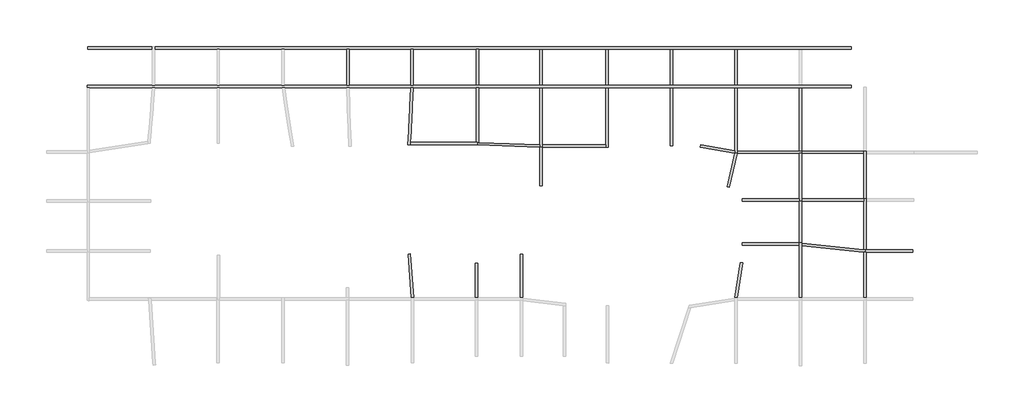
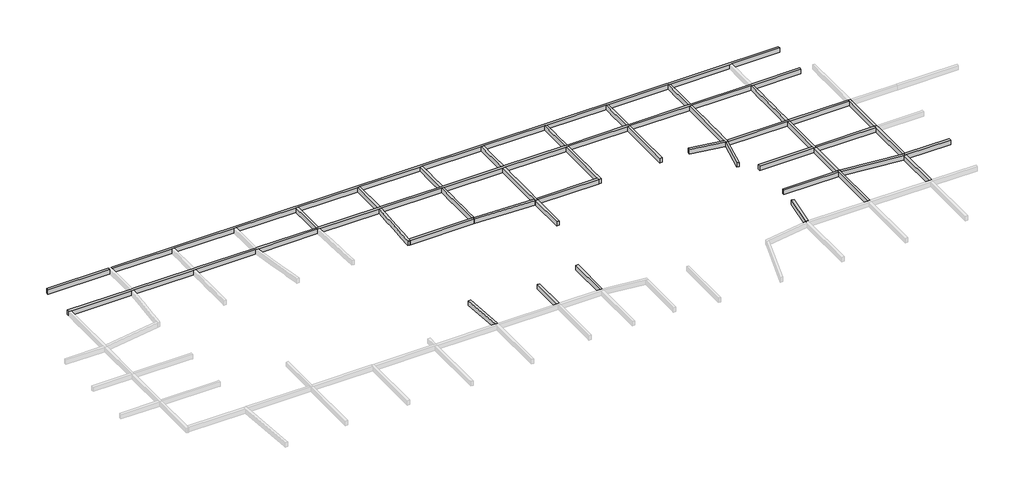
# One storey, part 7 of 8: 39 beams.
"""IFC4 building model written with IfcOpenShell, lengths in millimetres."""

from ifc_helpers import new_model, si_unit, frame, origin, place, context, project, spatial, polyline, outline, extrude, faceted_brep, element, save

model = new_model("IFC4")

# Units and contexts
model_context = context("Model", 3, world=origin())
ifc_project = project(units=[si_unit("LENGTHUNIT", "METRE", prefix="MILLI")], contexts=[model_context])

# Site, building, storey
site = spatial("IfcSite", under=ifc_project)
building = spatial("IfcBuilding", under=site)
storey = spatial("IfcBuildingStorey", under=building, Name="层高", Elevation=3300.0)

# Beams
placement = place(None, origin())
element("IfcBeam", 1, ObjectType="混凝土 - 矩形梁 : KL_beam", at=placement, inside=storey, context=model_context, shape_type="Brep", body=[
    faceted_brep([(155358.8476291, 153267.0451916, 3300.0), (155358.8476291, 152967.0451916, 3300.0), (155358.8476291, 152967.0451916, 2700.0), (155358.8476291, 153267.0451916, 2700.0), (149303.4366403, 153267.0451916, 3300.0), (149003.4366403, 153267.0451916, 3300.0), (141483.4366403, 153267.0451916, 3300.0), (141183.4366403, 153267.0451916, 3300.0), (133582.6046447, 153267.0451916, 3300.0), (133282.6046447, 153267.0451916, 3300.0), (125742.6046447, 153267.0451916, 3300.0), (125442.6046447, 153267.0451916, 3300.0), (117673.8474258, 153267.0451916, 3300.0), (117373.8474258, 153267.0451916, 3300.0), (109888.82396, 153267.0451916, 3300.0), (109588.82396, 153267.0451916, 3300.0), (101942.8755148, 153267.0451916, 3300.0), (101642.8755148, 153267.0451916, 3300.0), (94082.8755148, 153267.0451916, 3300.0), (93782.8755148, 153267.0451916, 3300.0), (86192.7452463, 153267.0451916, 3300.0), (85892.7452463, 153267.0451916, 3300.0), (78272.7452463, 153267.0451916, 3300.0), (77972.7452463, 153267.0451916, 3300.0), (70393.6976621, 153267.0451916, 3300.0), (70093.6976621, 153267.0451916, 3300.0), (62108.8476291, 153267.0451916, 3300.0), (62108.8476291, 152967.0451916, 3300.0), (62408.8476291, 152967.0451916, 3300.0), (70080.7837355, 152967.0451916, 3300.0), (70381.8074018, 152967.0451916, 3300.0), (77972.7452463, 152967.0451916, 3300.0), (78272.7452463, 152967.0451916, 3300.0), (85914.6331434, 152967.0451916, 3300.0), (86218.3726812, 152967.0451916, 3300.0), (93788.0221985, 152967.0451916, 3300.0), (94088.2050618, 152967.0451916, 3300.0), (101634.6906967, 152967.0451916, 3300.0), (101935.1141966, 152967.0451916, 3300.0), (109588.82396, 152967.0451916, 3300.0), (109888.82396, 152967.0451916, 3300.0), (117373.8474258, 152967.0451916, 3300.0), (117673.8474258, 152967.0451916, 3300.0), (125442.6046447, 152967.0451916, 3300.0), (125742.6046447, 152967.0451916, 3300.0), (133282.6046447, 152967.0451916, 3300.0), (133582.6046447, 152967.0451916, 3300.0), (141183.4366403, 152967.0451916, 3300.0), (141483.4366403, 152967.0451916, 3300.0), (149003.4366403, 152967.0451916, 3300.0), (149303.4366403, 152967.0451916, 3300.0), (62108.8476291, 152967.0451916, 2700.0), (62408.8476291, 152967.0451916, 2700.0), (70080.7837355, 152967.0451916, 2700.0), (70381.8074018, 152967.0451916, 2700.0), (77972.7452463, 152967.0451916, 2700.0), (78272.7452463, 152967.0451916, 2700.0), (85914.6331434, 152967.0451916, 2700.0), (86218.3726812, 152967.0451916, 2700.0), (93788.0221985, 152967.0451916, 2700.0), (94088.2050618, 152967.0451916, 2700.0), (101634.6906967, 152967.0451916, 2700.0), (101935.1141966, 152967.0451916, 2700.0), (109588.82396, 152967.0451916, 2700.0), (109888.82396, 152967.0451916, 2700.0), (117373.8474258, 152967.0451916, 2700.0), (117673.8474258, 152967.0451916, 2700.0), (125442.6046447, 152967.0451916, 2700.0), (125742.6046447, 152967.0451916, 2700.0), (133282.6046447, 152967.0451916, 2700.0), (133582.6046447, 152967.0451916, 2700.0), (141183.4366403, 152967.0451916, 2700.0), (141483.4366403, 152967.0451916, 2700.0), (149003.4366403, 152967.0451916, 2700.0), (149303.4366403, 152967.0451916, 2700.0), (62108.8476291, 153267.0451916, 2700.0), (70093.6976621, 153267.0451916, 2700.0), (70393.6976621, 153267.0451916, 2700.0), (77972.7452463, 153267.0451916, 2700.0), (78272.7452463, 153267.0451916, 2700.0), (85892.7452463, 153267.0451916, 2700.0), (86192.7452463, 153267.0451916, 2700.0), (93782.8755148, 153267.0451916, 2700.0), (94082.8755148, 153267.0451916, 2700.0), (101642.8755148, 153267.0451916, 2700.0), (101942.8755148, 153267.0451916, 2700.0), (109588.82396, 153267.0451916, 2700.0), (109888.82396, 153267.0451916, 2700.0), (117373.8474258, 153267.0451916, 2700.0), (117673.8474258, 153267.0451916, 2700.0), (125442.6046447, 153267.0451916, 2700.0), (125742.6046447, 153267.0451916, 2700.0), (133282.6046447, 153267.0451916, 2700.0), (133582.6046447, 153267.0451916, 2700.0), (141183.4366403, 153267.0451916, 2700.0), (141483.4366403, 153267.0451916, 2700.0), (149003.4366403, 153267.0451916, 2700.0), (149303.4366403, 153267.0451916, 2700.0)], [[[0, 1, 2, 3]], [[1, 0, 4, 5, 6, 7, 8, 9, 10, 11, 12, 13, 14, 15, 16, 17, 18, 19, 20, 21, 22, 23, 24, 25, 26, 27, 28, 29, 30, 31, 32, 33, 34, 35, 36, 37, 38, 39, 40, 41, 42, 43, 44, 45, 46, 47, 48, 49, 50]], [[2, 1, 50, 49, 48, 47, 46, 45, 44, 43, 42, 41, 40, 39, 38, 37, 36, 35, 34, 33, 32, 31, 30, 29, 28, 27, 51, 52, 53, 54, 55, 56, 57, 58, 59, 60, 61, 62, 63, 64, 65, 66, 67, 68, 69, 70, 71, 72, 73, 74]], [[3, 2, 74, 73, 72, 71, 70, 69, 68, 67, 66, 65, 64, 63, 62, 61, 60, 59, 58, 57, 56, 55, 54, 53, 52, 51, 75, 76, 77, 78, 79, 80, 81, 82, 83, 84, 85, 86, 87, 88, 89, 90, 91, 92, 93, 94, 95, 96, 97]], [[0, 3, 97, 96, 95, 94, 93, 92, 91, 90, 89, 88, 87, 86, 85, 84, 83, 82, 81, 80, 79, 78, 77, 76, 75, 26, 25, 24, 23, 22, 21, 20, 19, 18, 17, 16, 15, 14, 13, 12, 11, 10, 9, 8, 7, 6, 5, 4]], [[27, 26, 75, 51]]]),
])
element("IfcBeam", 2, ObjectType="混凝土 - 矩形梁 : KL_beam", at=placement, inside=storey, context=model_context, shape_type="Brep", body=[
    faceted_brep([(155398.8476291, 158006.8472847, 3300.0), (155398.8476291, 157706.8472847, 3300.0), (155398.8476291, 157706.8472847, 2700.0), (155398.8476291, 158006.8472847, 2700.0), (70393.6976621, 158006.8472847, 3300.0), (70393.6976621, 157706.8472847, 3300.0), (77972.7452463, 157706.8472847, 3300.0), (78272.7452463, 157706.8472847, 3300.0), (85892.7452463, 157706.8472847, 3300.0), (86192.7452463, 157706.8472847, 3300.0), (93782.8755148, 157706.8472847, 3300.0), (94082.8755148, 157706.8472847, 3300.0), (101642.8755148, 157706.8472847, 3300.0), (101942.8755148, 157706.8472847, 3300.0), (109588.82396, 157706.8472847, 3300.0), (109888.82396, 157706.8472847, 3300.0), (117373.8474258, 157706.8472847, 3300.0), (117673.8474258, 157706.8472847, 3300.0), (125442.6046447, 157706.8472847, 3300.0), (125742.6046447, 157706.8472847, 3300.0), (133282.6046447, 157706.8472847, 3300.0), (133582.6046447, 157706.8472847, 3300.0), (141183.4366403, 157706.8472847, 3300.0), (141483.4366403, 157706.8472847, 3300.0), (149003.4366403, 157706.8472847, 3300.0), (149303.4366403, 157706.8472847, 3300.0), (70393.6976621, 157706.8472847, 2700.0), (77972.7452463, 157706.8472847, 2700.0), (78272.7452463, 157706.8472847, 2700.0), (85892.7452463, 157706.8472847, 2700.0), (86192.7452463, 157706.8472847, 2700.0), (93782.8755148, 157706.8472847, 2700.0), (94082.8755148, 157706.8472847, 2700.0), (101642.8755148, 157706.8472847, 2700.0), (101942.8755148, 157706.8472847, 2700.0), (109588.82396, 157706.8472847, 2700.0), (109888.82396, 157706.8472847, 2700.0), (117373.8474258, 157706.8472847, 2700.0), (117673.8474258, 157706.8472847, 2700.0), (125442.6046447, 157706.8472847, 2700.0), (125742.6046447, 157706.8472847, 2700.0), (133282.6046447, 157706.8472847, 2700.0), (133582.6046447, 157706.8472847, 2700.0), (141183.4366403, 157706.8472847, 2700.0), (141483.4366403, 157706.8472847, 2700.0), (149003.4366403, 157706.8472847, 2700.0), (149303.4366403, 157706.8472847, 2700.0), (70393.6976621, 158006.8472847, 2700.0)], [[[0, 1, 2, 3]], [[1, 0, 4, 5, 6, 7, 8, 9, 10, 11, 12, 13, 14, 15, 16, 17, 18, 19, 20, 21, 22, 23, 24, 25]], [[2, 1, 25, 24, 23, 22, 21, 20, 19, 18, 17, 16, 15, 14, 13, 12, 11, 10, 9, 8, 7, 6, 5, 26, 27, 28, 29, 30, 31, 32, 33, 34, 35, 36, 37, 38, 39, 40, 41, 42, 43, 44, 45, 46]], [[3, 2, 46, 45, 44, 43, 42, 41, 40, 39, 38, 37, 36, 35, 34, 33, 32, 31, 30, 29, 28, 27, 26, 47]], [[0, 3, 47, 4]], [[5, 4, 47, 26]]]),
    faceted_brep([(62198.8476291, 158006.8472847, 3300.0), (62198.8476291, 158006.8472847, 2700.0), (62198.8476291, 157706.8472847, 2700.0), (62198.8476291, 157706.8472847, 3300.0), (70093.6976621, 158006.8472847, 3300.0), (70093.6976621, 157706.8472847, 3300.0), (70093.6976621, 157706.8472847, 2700.0), (70093.6976621, 158006.8472847, 2700.0)], [[[0, 1, 2, 3]], [[4, 5, 6, 7]], [[0, 3, 5, 4]], [[3, 2, 6, 5]], [[2, 1, 7, 6]], [[1, 0, 4, 7]]]),
])
element("IfcBeam", 3, ObjectType="混凝土 - 矩形梁 : KL_beam", at=placement, inside=storey, context=model_context, shape_type="Brep", body=[
    faceted_brep([(93782.8755148, 153267.0451916, 3300.0), (94082.8755148, 153267.0451916, 3300.0), (94082.8755148, 155366.9462381, 3300.0), (94082.8755148, 155766.9462381, 3300.0), (94082.8755148, 157706.8472847, 3300.0), (93782.8755148, 157706.8472847, 3300.0), (93782.8755148, 155766.9462381, 3300.0), (93782.8755148, 155366.9462381, 3300.0), (93782.8755148, 153267.0451916, 2700.0), (93782.8755148, 157706.8472847, 2700.0), (93782.8755148, 155766.9462381, 2700.0), (93782.8755148, 155366.9462381, 2700.0), (94082.8755148, 153267.0451916, 2700.0), (94082.8755148, 157706.8472847, 2700.0), (94082.8755148, 155766.9462381, 2700.0), (94082.8755148, 155366.9462381, 2700.0)], [[[0, 1, 2, 3, 4, 5, 6, 7]], [[8, 0, 7, 6, 5, 9, 10, 11]], [[12, 8, 11, 10, 9, 13, 14, 15]], [[1, 12, 15, 14, 13, 4, 3, 2]], [[1, 0, 8, 12]], [[5, 4, 13, 9]]]),
])
element("IfcBeam", 4, ObjectType="混凝土 - 矩形梁 : KL_beam", at=placement, inside=storey, context=model_context, shape_type="Brep", body=[
    faceted_brep([(101642.8755148, 153267.0451916, 3300.0), (101942.8755148, 153267.0451916, 3300.0), (101942.8755148, 155366.9462381, 3300.0), (101942.8755148, 155766.9462381, 3300.0), (101942.8755148, 157706.8472847, 3300.0), (101642.8755148, 157706.8472847, 3300.0), (101642.8755148, 155766.9462381, 3300.0), (101642.8755148, 155366.9462381, 3300.0), (101642.8755148, 153267.0451916, 2700.0), (101642.8755148, 157706.8472847, 2700.0), (101642.8755148, 155766.9462381, 2700.0), (101642.8755148, 155366.9462381, 2700.0), (101942.8755148, 153267.0451916, 2700.0), (101942.8755148, 157706.8472847, 2700.0), (101942.8755148, 155766.9462381, 2700.0), (101942.8755148, 155366.9462381, 2700.0)], [[[0, 1, 2, 3, 4, 5, 6, 7]], [[8, 0, 7, 6, 5, 9, 10, 11]], [[12, 8, 11, 10, 9, 13, 14, 15]], [[1, 12, 15, 14, 13, 4, 3, 2]], [[1, 0, 8, 12]], [[5, 4, 13, 9]]]),
])
element("IfcBeam", 5, ObjectType="混凝土 - 矩形梁 : KL_beam", at=placement, inside=storey, context=model_context, shape_type="Brep", body=[
    faceted_brep([(109588.82396, 153267.0451916, 3300.0), (109888.82396, 153267.0451916, 3300.0), (109888.82396, 155366.9462381, 3300.0), (109888.82396, 155766.9462381, 3300.0), (109888.82396, 157706.8472847, 3300.0), (109588.82396, 157706.8472847, 3300.0), (109588.82396, 155766.9462381, 3300.0), (109588.82396, 155366.9462381, 3300.0), (109588.82396, 153267.0451916, 2700.0), (109588.82396, 157706.8472847, 2700.0), (109588.82396, 155766.9462381, 2700.0), (109588.82396, 155366.9462381, 2700.0), (109888.82396, 153267.0451916, 2700.0), (109888.82396, 157706.8472847, 2700.0), (109888.82396, 155766.9462381, 2700.0), (109888.82396, 155366.9462381, 2700.0)], [[[0, 1, 2, 3, 4, 5, 6, 7]], [[8, 0, 7, 6, 5, 9, 10, 11]], [[12, 8, 11, 10, 9, 13, 14, 15]], [[1, 12, 15, 14, 13, 4, 3, 2]], [[1, 0, 8, 12]], [[5, 4, 13, 9]]]),
])
element("IfcBeam", 6, ObjectType="混凝土 - 矩形梁 : KL_beam", at=placement, inside=storey, context=model_context, shape_type="Brep", body=[
    faceted_brep([(117373.8474258, 153267.0451916, 3300.0), (117673.8474258, 153267.0451916, 3300.0), (117673.8474258, 155366.9462381, 3300.0), (117673.8474258, 155766.9462381, 3300.0), (117673.8474258, 157706.8472847, 3300.0), (117373.8474258, 157706.8472847, 3300.0), (117373.8474258, 155766.9462381, 3300.0), (117373.8474258, 155366.9462381, 3300.0), (117373.8474258, 153267.0451916, 2700.0), (117373.8474258, 157706.8472847, 2700.0), (117373.8474258, 155766.9462381, 2700.0), (117373.8474258, 155366.9462381, 2700.0), (117673.8474258, 153267.0451916, 2700.0), (117673.8474258, 157706.8472847, 2700.0), (117673.8474258, 155766.9462381, 2700.0), (117673.8474258, 155366.9462381, 2700.0)], [[[0, 1, 2, 3, 4, 5, 6, 7]], [[8, 0, 7, 6, 5, 9, 10, 11]], [[12, 8, 11, 10, 9, 13, 14, 15]], [[1, 12, 15, 14, 13, 4, 3, 2]], [[1, 0, 8, 12]], [[5, 4, 13, 9]]]),
])
element("IfcBeam", 7, ObjectType="混凝土 - 矩形梁 : KL_beam", at=placement, inside=storey, context=model_context, shape_type="Brep", body=[
    faceted_brep([(125442.6046447, 153267.0451916, 3300.0), (125742.6046447, 153267.0451916, 3300.0), (125742.6046447, 155366.9462381, 3300.0), (125742.6046447, 155766.9462381, 3300.0), (125742.6046447, 157706.8472847, 3300.0), (125442.6046447, 157706.8472847, 3300.0), (125442.6046447, 155766.9462381, 3300.0), (125442.6046447, 155366.9462381, 3300.0), (125442.6046447, 153267.0451916, 2700.0), (125442.6046447, 157706.8472847, 2700.0), (125442.6046447, 155766.9462381, 2700.0), (125442.6046447, 155366.9462381, 2700.0), (125742.6046447, 153267.0451916, 2700.0), (125742.6046447, 157706.8472847, 2700.0), (125742.6046447, 155766.9462381, 2700.0), (125742.6046447, 155366.9462381, 2700.0)], [[[0, 1, 2, 3, 4, 5, 6, 7]], [[8, 0, 7, 6, 5, 9, 10, 11]], [[12, 8, 11, 10, 9, 13, 14, 15]], [[1, 12, 15, 14, 13, 4, 3, 2]], [[1, 0, 8, 12]], [[5, 4, 13, 9]]]),
])
element("IfcBeam", 8, ObjectType="混凝土 - 矩形梁 : KL_beam", at=placement, inside=storey, context=model_context, shape_type="Brep", body=[
    faceted_brep([(133282.6046447, 153267.0451916, 3300.0), (133582.6046447, 153267.0451916, 3300.0), (133582.6046447, 155366.9462381, 3300.0), (133582.6046447, 155766.9462381, 3300.0), (133582.6046447, 157706.8472847, 3300.0), (133282.6046447, 157706.8472847, 3300.0), (133282.6046447, 155766.9462381, 3300.0), (133282.6046447, 155366.9462381, 3300.0), (133282.6046447, 153267.0451916, 2700.0), (133282.6046447, 157706.8472847, 2700.0), (133282.6046447, 155766.9462381, 2700.0), (133282.6046447, 155366.9462381, 2700.0), (133582.6046447, 153267.0451916, 2700.0), (133582.6046447, 157706.8472847, 2700.0), (133582.6046447, 155766.9462381, 2700.0), (133582.6046447, 155366.9462381, 2700.0)], [[[0, 1, 2, 3, 4, 5, 6, 7]], [[8, 0, 7, 6, 5, 9, 10, 11]], [[12, 8, 11, 10, 9, 13, 14, 15]], [[1, 12, 15, 14, 13, 4, 3, 2]], [[1, 0, 8, 12]], [[5, 4, 13, 9]]]),
])
element("IfcBeam", 9, ObjectType="混凝土 - 矩形梁 : KL_beam", at=placement, inside=storey, context=model_context, shape_type="Brep", body=[
    faceted_brep([(141183.4366403, 153267.0451916, 3300.0), (141483.4366403, 153267.0451916, 3300.0), (141483.4366403, 155366.9462381, 3300.0), (141483.4366403, 155766.9462381, 3300.0), (141483.4366403, 157706.8472847, 3300.0), (141183.4366403, 157706.8472847, 3300.0), (141183.4366403, 155766.9462381, 3300.0), (141183.4366403, 155366.9462381, 3300.0), (141183.4366403, 153267.0451916, 2700.0), (141183.4366403, 157706.8472847, 2700.0), (141183.4366403, 155766.9462381, 2700.0), (141183.4366403, 155366.9462381, 2700.0), (141483.4366403, 153267.0451916, 2700.0), (141483.4366403, 157706.8472847, 2700.0), (141483.4366403, 155766.9462381, 2700.0), (141483.4366403, 155366.9462381, 2700.0)], [[[0, 1, 2, 3, 4, 5, 6, 7]], [[8, 0, 7, 6, 5, 9, 10, 11]], [[12, 8, 11, 10, 9, 13, 14, 15]], [[1, 12, 15, 14, 13, 4, 3, 2]], [[1, 0, 8, 12]], [[5, 4, 13, 9]]]),
])
element("IfcBeam", 10, ObjectType="混凝土 - 矩形梁 : KL_beam", at=placement, inside=storey, context=model_context, shape_type="Brep", body=[
    faceted_brep([(101286.0486898, 132683.0858933, 3300.0), (101585.3179049, 132704.0128354, 3300.0), (101585.3179049, 132704.0128354, 2700.0), (101286.0486898, 132683.0858933, 2700.0), (101659.9672049, 127335.802002, 3300.0), (101670.8225114, 127335.802002, 3300.0), (101960.6997743, 127335.802002, 3300.0), (101960.6997743, 127335.802002, 2700.0), (101670.8225114, 127335.802002, 2700.0), (101659.9672049, 127335.802002, 2700.0)], [[[0, 1, 2, 3]], [[1, 0, 4, 5, 6]], [[2, 1, 6, 7]], [[3, 2, 7, 8, 9]], [[0, 3, 9, 4]], [[4, 9, 8, 7, 6, 5]]]),
    faceted_brep([(101981.6778179, 127035.802002, 2700.0), (101981.6778179, 127035.802002, 3300.0), (101970.8225114, 127035.802002, 3300.0), (101970.8225114, 127035.802002, 2700.0), (101970.8225114, 127191.0401174, 3300.0), (101970.8225114, 127191.0401174, 2700.0)], [[[0, 1, 2, 3]], [[2, 4, 5, 3]], [[1, 4, 2]], [[1, 0, 5, 4]], [[5, 0, 3]]]),
])
element("IfcBeam", 11, ObjectType="混凝土 - 矩形梁 : KL_beam", at=placement, inside=storey, context=model_context, shape_type="SweptSolid", body=[
    extrude(outline(polyline([(109470.8225114, 131593.2738066), (109770.8225114, 131593.2738066), (109770.8225114, 127335.802002), (109470.8225114, 127335.802002), (109470.8225114, 131593.2738066)])), frame((0.0, 0.0, 2700.0), z_axis=(0.0, 0.0, 1.0), x_axis=(1.0, 0.0, 0.0)), (0.0, 0.0, 1.0), 600.0),
])
element("IfcBeam", 12, ObjectType="混凝土 - 矩形梁 : KL_beam", at=placement, inside=storey, context=model_context, shape_type="SweptSolid", body=[
    extrude(outline(polyline([(114973.8238915, 132693.2738046), (115273.8238915, 132693.2738046), (115273.8238915, 127335.802002), (114973.8238915, 127335.802002), (114973.8238915, 132693.2738046)])), frame((0.0, 0.0, 2700.0), z_axis=(0.0, 0.0, 1.0), x_axis=(1.0, 0.0, 0.0)), (0.0, 0.0, 1.0), 600.0),
])
element("IfcBeam", 13, ObjectType="混凝土 - 矩形梁 : KL_beam", at=placement, inside=storey, context=model_context, shape_type="Brep", body=[
    faceted_brep([(149348.8238805, 134044.1147453, 3300.0), (149303.4366403, 134044.1147453, 3300.0), (149206.6850474, 134044.1147453, 3300.0), (149048.8238805, 134044.1147453, 3300.0), (149048.8238805, 133744.1147453, 3300.0), (149048.8238805, 127344.1147453, 3300.0), (149348.8238805, 127344.1147453, 3300.0), (149348.8238805, 133727.5228681, 3300.0), (149348.8238805, 134029.175352, 3300.0), (149348.8238805, 134044.1147453, 2700.0), (149348.8238805, 127344.1147453, 2700.0), (149348.8238805, 133727.5228681, 2700.0), (149348.8238805, 134029.175352, 2700.0), (149048.8238805, 134044.1147453, 2700.0), (149206.6850474, 134044.1147453, 2700.0), (149303.4366403, 134044.1147453, 2700.0), (149048.8238805, 127344.1147453, 2700.0), (149048.8238805, 133744.1147453, 2700.0)], [[[0, 1, 2, 3, 4, 5, 6, 7, 8]], [[9, 0, 8, 7, 6, 10, 11, 12]], [[13, 14, 15, 9, 12, 11, 10, 16, 17]], [[3, 13, 17, 16, 5, 4]], [[6, 5, 16, 10]], [[3, 2, 1, 0, 9, 15, 14, 13]]]),
])
element("IfcBeam", 14, ObjectType="混凝土 - 矩形梁 : KL_beam", at=placement, inside=storey, context=model_context, shape_type="Brep", body=[
    faceted_brep([(141854.6257221, 131662.1774478, 3300.0), (142150.9322243, 131615.2471082, 3300.0), (142150.9322243, 131615.2471082, 2700.0), (141854.6257221, 131662.1774478, 2700.0), (141170.7117777, 127344.1147453, 3300.0), (141448.8238805, 127344.1147453, 3300.0), (141474.4513154, 127344.1147453, 3300.0), (141474.4513154, 127344.1147453, 2700.0), (141448.8238805, 127344.1147453, 2700.0), (141170.7117777, 127344.1147453, 2700.0)], [[[0, 1, 2, 3]], [[1, 0, 4, 5, 6]], [[2, 1, 6, 7]], [[3, 2, 7, 8, 9]], [[0, 3, 9, 4]], [[4, 9, 8, 7, 6, 5]]]),
    faceted_brep([(141118.3137403, 127013.2865575, 3300.0), (141118.3137403, 127013.2865575, 2700.0), (141148.8238805, 127018.1739614, 2700.0), (141148.8238805, 127018.1739614, 3300.0), (141148.8238805, 127205.9200013, 2700.0), (141148.8238805, 127205.9200013, 3300.0), (141148.8238805, 127044.1147453, 3300.0), (141148.8238805, 127044.1147453, 2700.0)], [[[0, 1, 2, 3]], [[4, 5, 6, 3, 2, 7]], [[5, 0, 3, 6]], [[1, 4, 7, 2]], [[1, 0, 5, 4]]]),
])
element("IfcBeam", 15, ObjectType="混凝土 - 矩形梁 : KL_beam", at=placement, inside=storey, context=model_context, shape_type="Brep", body=[
    faceted_brep([(142092.714265, 133744.1147453, 3300.0), (142092.714265, 134044.1147453, 3300.0), (142092.714265, 134044.1147453, 2700.0), (142092.714265, 133744.1147453, 2700.0), (149048.8238805, 133744.1147453, 3300.0), (149048.8238805, 134044.1147453, 3300.0), (149044.6739148, 134044.1147453, 3300.0), (149003.4366403, 134044.1147453, 3300.0), (149048.8238805, 134044.1147453, 2700.0), (149044.6739148, 134044.1147453, 2700.0), (149003.4366403, 134044.1147453, 2700.0), (149048.8238805, 133744.1147453, 2700.0)], [[[0, 1, 2, 3]], [[1, 0, 4, 5, 6, 7]], [[2, 1, 7, 6, 5, 8, 9, 10]], [[3, 2, 10, 9, 8, 11]], [[0, 3, 11, 4]], [[5, 4, 11, 8]]]),
])
element("IfcBeam", 16, ObjectType="混凝土 - 矩形梁 : KL_beam", at=placement, inside=storey, context=model_context, shape_type="Brep", body=[
    faceted_brep([(149348.8238805, 133727.5228681, 3300.0), (156905.5468539, 132933.2792789, 3300.0), (157047.685687, 132918.3398855, 3300.0), (157063.4080208, 133218.3398855, 3300.0), (156905.5468539, 133234.9317627, 3300.0), (149348.8238805, 134029.175352, 3300.0), (149348.8238805, 133744.1147453, 3300.0), (149348.8238805, 133727.5228681, 2700.0), (156905.5468539, 132933.2792789, 2700.0), (157047.685687, 132918.3398855, 2700.0), (149348.8238805, 133744.1147453, 2700.0), (149348.8238805, 134029.175352, 2700.0), (156905.5468539, 133234.9317627, 2700.0), (157063.4080208, 133218.3398855, 2700.0)], [[[0, 1, 2, 3, 4, 5, 6]], [[2, 1, 0, 7, 8, 9]], [[9, 8, 7, 10, 11, 12, 13]], [[11, 5, 4, 3, 13, 12]], [[7, 0, 6, 5, 11, 10]], [[3, 2, 9, 13]]]),
    faceted_brep([(149046.4440807, 134060.9567496, 3300.0), (149046.4440807, 134060.9567496, 2700.0), (149044.6739148, 134044.1147453, 2700.0), (149044.6739148, 134044.1147453, 3300.0), (149048.8238805, 134044.1147453, 2700.0), (149206.6850474, 134044.1147453, 2700.0), (149206.6850474, 134044.1147453, 3300.0), (149048.8238805, 134044.1147453, 3300.0)], [[[0, 1, 2, 3]], [[3, 2, 4, 5, 6, 7]], [[3, 7, 6, 0]], [[5, 4, 2, 1]], [[1, 0, 6, 5]]]),
])
element("IfcBeam", 17, ObjectType="混凝土 - 矩形梁 : KL_beam", at=placement, inside=storey, context=model_context, shape_type="Brep", body=[
    faceted_brep([(162873.6972933, 133218.3398855, 3300.0), (162873.6972933, 132918.3398855, 3300.0), (162873.6972933, 132918.3398855, 2700.0), (162873.6972933, 133218.3398855, 2700.0), (157205.5468539, 133218.3398855, 3300.0), (157063.4080208, 133218.3398855, 3300.0), (157047.685687, 132918.3398855, 3300.0), (157205.5468539, 132918.3398855, 3300.0), (157047.685687, 132918.3398855, 2700.0), (157205.5468539, 132918.3398855, 2700.0), (157063.4080208, 133218.3398855, 2700.0), (157205.5468539, 133218.3398855, 2700.0)], [[[0, 1, 2, 3]], [[1, 0, 4, 5, 6, 7]], [[2, 1, 7, 6, 8, 9]], [[3, 2, 9, 8, 10, 11]], [[0, 3, 11, 10, 5, 4]], [[5, 10, 8, 6]]]),
])
element("IfcBeam", 18, ObjectType="混凝土 - 矩形梁 : KL_beam", at=placement, inside=storey, context=model_context, shape_type="SweptSolid", body=[
    extrude(outline(polyline([(157205.5468539, 127344.1147453), (156905.5468539, 127344.1147453), (156905.5468539, 132933.2792789), (157047.685687, 132918.3398855), (157205.5468539, 132918.3398855), (157205.5468539, 127344.1147453)])), frame((0.0, 0.0, 2700.0), z_axis=(0.0, 0.0, 1.0), x_axis=(1.0, 0.0, 0.0)), (0.0, 0.0, 1.0), 600.0),
])
element("IfcBeam", 19, ObjectType="混凝土 - 矩形梁 : KL_beam", at=placement, inside=storey, context=model_context, shape_type="Brep", body=[
    faceted_brep([(156905.5468539, 133234.9317627, 3300.0), (157063.4080208, 133218.3398855, 3300.0), (157205.5468539, 133218.3398855, 3300.0), (157205.5468539, 139118.3398855, 3300.0), (157205.5468539, 139418.3398855, 3300.0), (156905.5468539, 139418.3398855, 3300.0), (156905.5468539, 139118.3398855, 3300.0), (157205.5468539, 133218.3398855, 2700.0), (157205.5468539, 139118.3398855, 2700.0), (157205.5468539, 139418.3398855, 2700.0), (157063.4080208, 133218.3398855, 2700.0), (156905.5468539, 133234.9317627, 2700.0), (156905.5468539, 139118.3398855, 2700.0), (156905.5468539, 139418.3398855, 2700.0)], [[[0, 1, 2, 3, 4, 5, 6]], [[2, 7, 8, 9, 4, 3]], [[10, 11, 12, 13, 9, 8, 7]], [[11, 0, 6, 5, 13, 12]], [[1, 0, 11, 10]], [[2, 1, 10, 7]], [[5, 4, 9, 13]]]),
])
element("IfcBeam", 20, ObjectType="混凝土 - 矩形梁 : KL_beam", at=placement, inside=storey, context=model_context, shape_type="Brep", body=[
    faceted_brep([(157205.5468539, 145218.3398855, 3300.0), (156905.5468539, 145218.3398855, 3300.0), (156905.5468539, 144967.0451916, 3300.0), (156905.5468539, 139418.3398855, 3300.0), (157205.5468539, 139418.3398855, 3300.0), (157205.5468539, 144918.3398855, 3300.0), (157205.5468539, 145218.3398855, 2700.0), (157205.5468539, 139418.3398855, 2700.0), (157205.5468539, 144918.3398855, 2700.0), (156905.5468539, 145218.3398855, 2700.0), (156905.5468539, 139418.3398855, 2700.0), (156905.5468539, 144967.0451916, 2700.0)], [[[0, 1, 2, 3, 4, 5]], [[6, 0, 5, 4, 7, 8]], [[9, 6, 8, 7, 10, 11]], [[1, 9, 11, 10, 3, 2]], [[1, 0, 6, 9]], [[4, 3, 10, 7]]]),
])
element("IfcBeam", 21, ObjectType="混凝土 - 矩形梁 : KL_beam", at=placement, inside=storey, context=model_context, shape_type="Brep", body=[
    faceted_brep([(101265.6115787, 146023.4361595, 3300.0), (101565.1886759, 146007.5125022, 3300.0), (101581.1348121, 146307.5125022, 3300.0), (101652.7187262, 147654.2446479, 3300.0), (101673.9802411, 148054.2446479, 3300.0), (101799.0194755, 150406.6496336, 3300.0), (101820.2809905, 150806.6496336, 3300.0), (101935.1141966, 152967.0451916, 3300.0), (101634.6906967, 152967.0451916, 3300.0), (101519.8574906, 150806.6496336, 3300.0), (101498.5959757, 150406.6496336, 3300.0), (101373.5567413, 148054.2446479, 3300.0), (101352.2952263, 147654.2446479, 3300.0), (101265.6115787, 146023.4361595, 2700.0), (101634.6906967, 152967.0451916, 2700.0), (101519.8574906, 150806.6496336, 2700.0), (101498.5959757, 150406.6496336, 2700.0), (101373.5567413, 148054.2446479, 2700.0), (101352.2952263, 147654.2446479, 2700.0), (101565.1886759, 146007.5125022, 2700.0), (101935.1141966, 152967.0451916, 2700.0), (101820.2809905, 150806.6496336, 2700.0), (101799.0194755, 150406.6496336, 2700.0), (101673.9802411, 148054.2446479, 2700.0), (101652.7187262, 147654.2446479, 2700.0), (101581.1348121, 146307.5125022, 2700.0)], [[[0, 1, 2, 3, 4, 5, 6, 7, 8, 9, 10, 11, 12]], [[13, 0, 12, 11, 10, 9, 8, 14, 15, 16, 17, 18]], [[19, 13, 18, 17, 16, 15, 14, 20, 21, 22, 23, 24, 25]], [[1, 19, 25, 24, 23, 22, 21, 20, 7, 6, 5, 4, 3, 2]], [[8, 7, 20, 14]], [[1, 0, 13, 19]]]),
])
element("IfcBeam", 22, ObjectType="混凝土 - 矩形梁 : KL_beam", at=placement, inside=storey, context=model_context, shape_type="Brep", body=[
    faceted_brep([(109888.82396, 152967.0451916, 3300.0), (109588.82396, 152967.0451916, 3300.0), (109588.82396, 150806.6496336, 3300.0), (109588.82396, 150406.6496336, 3300.0), (109588.82396, 148054.2446479, 3300.0), (109588.82396, 147654.2446479, 3300.0), (109588.82396, 146307.5125022, 3300.0), (109731.2172347, 146307.5125022, 3300.0), (109888.82396, 146302.0087541, 3300.0), (109888.82396, 147654.2446479, 3300.0), (109888.82396, 148054.2446479, 3300.0), (109888.82396, 150406.6496336, 3300.0), (109888.82396, 150806.6496336, 3300.0), (109588.82396, 152967.0451916, 2700.0), (109588.82396, 150806.6496336, 2700.0), (109588.82396, 150406.6496336, 2700.0), (109588.82396, 148054.2446479, 2700.0), (109588.82396, 147654.2446479, 2700.0), (109588.82396, 146307.5125022, 2700.0), (109888.82396, 152967.0451916, 2700.0), (109888.82396, 150806.6496336, 2700.0), (109888.82396, 150406.6496336, 2700.0), (109888.82396, 148054.2446479, 2700.0), (109888.82396, 147654.2446479, 2700.0), (109888.82396, 146302.0087541, 2700.0), (109731.2172347, 146307.5125022, 2700.0)], [[[0, 1, 2, 3, 4, 5, 6, 7, 8, 9, 10, 11, 12]], [[1, 13, 14, 15, 16, 17, 18, 6, 5, 4, 3, 2]], [[13, 19, 20, 21, 22, 23, 24, 25, 18, 17, 16, 15, 14]], [[19, 0, 12, 11, 10, 9, 8, 24, 23, 22, 21, 20]], [[1, 0, 19, 13]], [[8, 7, 25, 24]], [[7, 6, 18, 25]]]),
])
element("IfcBeam", 23, ObjectType="混凝土 - 矩形梁 : KL_beam", at=placement, inside=storey, context=model_context, shape_type="Brep", body=[
    faceted_brep([(117373.8474258, 145735.2964279, 3300.0), (117673.8474258, 145735.2964279, 3300.0), (117673.8474258, 146035.2964279, 3300.0), (117673.8474258, 147654.2446479, 3300.0), (117673.8474258, 148054.2446479, 3300.0), (117673.8474258, 150406.6496336, 3300.0), (117673.8474258, 150806.6496336, 3300.0), (117673.8474258, 152967.0451916, 3300.0), (117373.8474258, 152967.0451916, 3300.0), (117373.8474258, 150806.6496336, 3300.0), (117373.8474258, 150406.6496336, 3300.0), (117373.8474258, 148054.2446479, 3300.0), (117373.8474258, 147654.2446479, 3300.0), (117373.8474258, 146040.625975, 3300.0), (117373.8474258, 145740.4431117, 3300.0), (117373.8474258, 145735.2964279, 2700.0), (117373.8474258, 152967.0451916, 2700.0), (117373.8474258, 150806.6496336, 2700.0), (117373.8474258, 150406.6496336, 2700.0), (117373.8474258, 148054.2446479, 2700.0), (117373.8474258, 147654.2446479, 2700.0), (117373.8474258, 146040.625975, 2700.0), (117373.8474258, 145740.4431117, 2700.0), (117673.8474258, 145735.2964279, 2700.0), (117673.8474258, 152967.0451916, 2700.0), (117673.8474258, 150806.6496336, 2700.0), (117673.8474258, 150406.6496336, 2700.0), (117673.8474258, 148054.2446479, 2700.0), (117673.8474258, 147654.2446479, 2700.0), (117673.8474258, 146035.2964279, 2700.0)], [[[0, 1, 2, 3, 4, 5, 6, 7, 8, 9, 10, 11, 12, 13, 14]], [[15, 0, 14, 13, 12, 11, 10, 9, 8, 16, 17, 18, 19, 20, 21, 22]], [[23, 15, 22, 21, 20, 19, 18, 17, 16, 24, 25, 26, 27, 28, 29]], [[1, 23, 29, 28, 27, 26, 25, 24, 7, 6, 5, 4, 3, 2]], [[8, 7, 24, 16]], [[1, 0, 15, 23]]]),
])
element("IfcBeam", 24, ObjectType="混凝土 - 矩形梁 : KL_beam", at=placement, inside=storey, context=model_context, shape_type="SweptSolid", body=[
    extrude(outline(polyline([(117673.8474258, 141044.2705383), (117373.8474258, 141044.2705383), (117373.8474258, 145735.2964279), (117673.8474258, 145735.2964279), (117673.8474258, 141044.2705383)])), frame((0.0, 0.0, 2700.0), z_axis=(0.0, 0.0, 1.0), x_axis=(1.0, 0.0, 0.0)), (0.0, 0.0, 1.0), 600.0),
])
element("IfcBeam", 25, ObjectType="混凝土 - 矩形梁 : KL_beam", at=placement, inside=storey, context=model_context, shape_type="Brep", body=[
    faceted_brep([(125442.6046447, 145735.2964279, 3300.0), (125742.6046447, 145735.2964279, 3300.0), (125742.6046447, 147654.2446479, 3300.0), (125742.6046447, 148054.2446479, 3300.0), (125742.6046447, 150406.6496336, 3300.0), (125742.6046447, 150806.6496336, 3300.0), (125742.6046447, 152967.0451916, 3300.0), (125442.6046447, 152967.0451916, 3300.0), (125442.6046447, 150806.6496336, 3300.0), (125442.6046447, 150406.6496336, 3300.0), (125442.6046447, 148054.2446479, 3300.0), (125442.6046447, 147654.2446479, 3300.0), (125442.6046447, 146035.2964279, 3300.0), (125442.6046447, 145735.2964279, 2700.0), (125442.6046447, 152967.0451916, 2700.0), (125442.6046447, 150806.6496336, 2700.0), (125442.6046447, 150406.6496336, 2700.0), (125442.6046447, 148054.2446479, 2700.0), (125442.6046447, 147654.2446479, 2700.0), (125442.6046447, 146035.2964279, 2700.0), (125742.6046447, 145735.2964279, 2700.0), (125742.6046447, 152967.0451916, 2700.0), (125742.6046447, 150806.6496336, 2700.0), (125742.6046447, 150406.6496336, 2700.0), (125742.6046447, 148054.2446479, 2700.0), (125742.6046447, 147654.2446479, 2700.0)], [[[0, 1, 2, 3, 4, 5, 6, 7, 8, 9, 10, 11, 12]], [[13, 0, 12, 11, 10, 9, 8, 7, 14, 15, 16, 17, 18, 19]], [[20, 13, 19, 18, 17, 16, 15, 14, 21, 22, 23, 24, 25]], [[1, 20, 25, 24, 23, 22, 21, 6, 5, 4, 3, 2]], [[7, 6, 21, 14]], [[1, 0, 13, 20]]]),
])
element("IfcBeam", 26, ObjectType="混凝土 - 矩形梁 : KL_beam", at=placement, inside=storey, context=model_context, shape_type="Brep", body=[
    faceted_brep([(133582.6046447, 145885.6708097, 3300.0), (133282.6046447, 145885.6708097, 3300.0), (133282.6046447, 145885.6708097, 2700.0), (133582.6046447, 145885.6708097, 2700.0), (133582.6046447, 147654.2446479, 3300.0), (133582.6046447, 148054.2446479, 3300.0), (133582.6046447, 150406.6496336, 3300.0), (133582.6046447, 150806.6496336, 3300.0), (133582.6046447, 152967.0451916, 3300.0), (133282.6046447, 152967.0451916, 3300.0), (133282.6046447, 150806.6496336, 3300.0), (133282.6046447, 150406.6496336, 3300.0), (133282.6046447, 148054.2446479, 3300.0), (133282.6046447, 147654.2446479, 3300.0), (133282.6046447, 152967.0451916, 2700.0), (133282.6046447, 150806.6496336, 2700.0), (133282.6046447, 150406.6496336, 2700.0), (133282.6046447, 148054.2446479, 2700.0), (133282.6046447, 147654.2446479, 2700.0), (133582.6046447, 152967.0451916, 2700.0), (133582.6046447, 150806.6496336, 2700.0), (133582.6046447, 150406.6496336, 2700.0), (133582.6046447, 148054.2446479, 2700.0), (133582.6046447, 147654.2446479, 2700.0)], [[[0, 1, 2, 3]], [[1, 0, 4, 5, 6, 7, 8, 9, 10, 11, 12, 13]], [[2, 1, 13, 12, 11, 10, 9, 14, 15, 16, 17, 18]], [[3, 2, 18, 17, 16, 15, 14, 19, 20, 21, 22, 23]], [[0, 3, 23, 22, 21, 20, 19, 8, 7, 6, 5, 4]], [[9, 8, 19, 14]]]),
])
element("IfcBeam", 27, ObjectType="混凝土 - 矩形梁 : KL_beam", at=placement, inside=storey, context=model_context, shape_type="Brep", body=[
    faceted_brep([(141183.4366403, 144991.2614678, 3300.0), (141483.4366403, 144991.2614678, 3300.0), (141483.4366403, 145267.0451916, 3300.0), (141483.4366403, 147654.2446479, 3300.0), (141483.4366403, 148054.2446479, 3300.0), (141483.4366403, 150406.6496336, 3300.0), (141483.4366403, 150806.6496336, 3300.0), (141483.4366403, 152967.0451916, 3300.0), (141183.4366403, 152967.0451916, 3300.0), (141183.4366403, 150806.6496336, 3300.0), (141183.4366403, 150406.6496336, 3300.0), (141183.4366403, 148054.2446479, 3300.0), (141183.4366403, 147654.2446479, 3300.0), (141183.4366403, 145295.9236611, 3300.0), (141183.4366403, 144991.2614678, 2700.0), (141183.4366403, 152967.0451916, 2700.0), (141183.4366403, 150806.6496336, 2700.0), (141183.4366403, 150406.6496336, 2700.0), (141183.4366403, 148054.2446479, 2700.0), (141183.4366403, 147654.2446479, 2700.0), (141183.4366403, 145295.9236611, 2700.0), (141483.4366403, 144991.2614678, 2700.0), (141483.4366403, 152967.0451916, 2700.0), (141483.4366403, 150806.6496336, 2700.0), (141483.4366403, 150406.6496336, 2700.0), (141483.4366403, 148054.2446479, 2700.0), (141483.4366403, 147654.2446479, 2700.0), (141483.4366403, 145267.0451916, 2700.0)], [[[0, 1, 2, 3, 4, 5, 6, 7, 8, 9, 10, 11, 12, 13]], [[14, 0, 13, 12, 11, 10, 9, 8, 15, 16, 17, 18, 19, 20]], [[21, 14, 20, 19, 18, 17, 16, 15, 22, 23, 24, 25, 26, 27]], [[1, 21, 27, 26, 25, 24, 23, 22, 7, 6, 5, 4, 3, 2]], [[8, 7, 22, 15]], [[1, 0, 14, 21]]]),
])
element("IfcBeam", 28, ObjectType="混凝土 - 矩形梁 : KL_beam", at=placement, inside=storey, context=model_context, shape_type="Brep", body=[
    faceted_brep([(137018.8891994, 146032.9756187, 3300.0), (137018.8891994, 146032.9756187, 2700.0), (136966.6069535, 145737.5664673, 2700.0), (136966.6069535, 145737.5664673, 3300.0), (141151.7464142, 144996.8700828, 3300.0), (141183.4366403, 144991.2614678, 3300.0), (141183.4366403, 145295.9236611, 3300.0), (141151.7464142, 144996.8700828, 2700.0), (141183.4366403, 144991.2614678, 2700.0), (141183.4366403, 145295.9236611, 2700.0)], [[[0, 1, 2, 3]], [[0, 3, 4, 5, 6]], [[3, 2, 7, 8, 5, 4]], [[2, 1, 9, 8, 7]], [[1, 0, 6, 9]], [[6, 5, 8, 9]]]),
])
element("IfcBeam", 29, ObjectType="混凝土 - 矩形梁 : KL_beam", at=placement, inside=storey, context=model_context, shape_type="Brep", body=[
    faceted_brep([(141483.4366403, 144991.2614678, 3300.0), (141183.4366403, 144991.2614678, 3300.0), (141151.7464142, 144996.8700828, 3300.0), (141144.8607955, 144967.0451916, 3300.0), (141452.7520278, 144967.0451916, 3300.0), (149003.4366403, 144967.0451916, 3300.0), (149303.4366403, 144967.0451916, 3300.0), (149303.4366403, 145267.0451916, 3300.0), (149003.4366403, 145267.0451916, 3300.0), (141483.4366403, 145267.0451916, 3300.0), (141483.4366403, 145242.8289154, 3300.0), (141144.8607955, 144967.0451916, 2700.0), (141452.7520278, 144967.0451916, 2700.0), (149003.4366403, 144967.0451916, 2700.0), (149303.4366403, 144967.0451916, 2700.0), (141183.4366403, 144991.2614678, 2700.0), (141483.4366403, 144991.2614678, 2700.0), (141483.4366403, 145242.8289154, 2700.0), (141483.4366403, 145267.0451916, 2700.0), (149003.4366403, 145267.0451916, 2700.0), (149303.4366403, 145267.0451916, 2700.0), (141151.7464142, 144996.8700828, 2700.0)], [[[0, 1, 2, 3, 4, 5, 6, 7, 8, 9, 10]], [[3, 11, 12, 13, 14, 6, 5, 4]], [[15, 16, 17, 18, 19, 20, 14, 13, 12, 11, 21]], [[18, 9, 8, 7, 20, 19]], [[11, 3, 2, 21]], [[16, 0, 10, 9, 18, 17]], [[0, 16, 15, 1]], [[2, 1, 15, 21]], [[7, 6, 14, 20]]]),
])
element("IfcBeam", 30, ObjectType="混凝土 - 矩形梁 : KL_beam", at=placement, inside=storey, context=model_context, shape_type="Brep", body=[
    faceted_brep([(156905.5468539, 144967.0451916, 3300.0), (156905.5468539, 145218.3398855, 3300.0), (156905.5468539, 145267.0451916, 3300.0), (149303.4366403, 145267.0451916, 3300.0), (149303.4366403, 144967.0451916, 3300.0), (156905.5468539, 144967.0451916, 2700.0), (149303.4366403, 144967.0451916, 2700.0), (156905.5468539, 145267.0451916, 2700.0), (156905.5468539, 145218.3398855, 2700.0), (149303.4366403, 145267.0451916, 2700.0)], [[[0, 1, 2, 3, 4]], [[5, 0, 4, 6]], [[7, 8, 5, 6, 9]], [[2, 7, 9, 3]], [[0, 5, 8, 7, 2, 1]], [[4, 3, 9, 6]]]),
])
element("IfcBeam", 31, ObjectType="混凝土 - 矩形梁 : KL_beam", at=placement, inside=storey, context=model_context, shape_type="Brep", body=[
    faceted_brep([(149003.4366403, 145267.0451916, 3300.0), (149303.4366403, 145267.0451916, 3300.0), (149303.4366403, 147654.2446479, 3300.0), (149303.4366403, 148054.2446479, 3300.0), (149303.4366403, 150406.6496336, 3300.0), (149303.4366403, 150806.6496336, 3300.0), (149303.4366403, 152967.0451916, 3300.0), (149003.4366403, 152967.0451916, 3300.0), (149003.4366403, 150806.6496336, 3300.0), (149003.4366403, 150406.6496336, 3300.0), (149003.4366403, 148054.2446479, 3300.0), (149003.4366403, 147654.2446479, 3300.0), (149003.4366403, 145267.0451916, 2700.0), (149003.4366403, 152967.0451916, 2700.0), (149003.4366403, 150806.6496336, 2700.0), (149003.4366403, 150406.6496336, 2700.0), (149003.4366403, 148054.2446479, 2700.0), (149003.4366403, 147654.2446479, 2700.0), (149303.4366403, 145267.0451916, 2700.0), (149303.4366403, 152967.0451916, 2700.0), (149303.4366403, 150806.6496336, 2700.0), (149303.4366403, 150406.6496336, 2700.0), (149303.4366403, 148054.2446479, 2700.0), (149303.4366403, 147654.2446479, 2700.0)], [[[0, 1, 2, 3, 4, 5, 6, 7, 8, 9, 10, 11]], [[12, 0, 11, 10, 9, 8, 7, 13, 14, 15, 16, 17]], [[18, 12, 17, 16, 15, 14, 13, 19, 20, 21, 22, 23]], [[1, 18, 23, 22, 21, 20, 19, 6, 5, 4, 3, 2]], [[1, 0, 12, 18]], [[7, 6, 19, 13]]]),
])
element("IfcBeam", 32, ObjectType="混凝土 - 矩形梁 : KL_beam", at=placement, inside=storey, context=model_context, shape_type="Brep", body=[
    faceted_brep([(149003.4366403, 139118.3398855, 3300.0), (149303.4366403, 139118.3398855, 3300.0), (149303.4366403, 139418.3398855, 3300.0), (149303.4366403, 144967.0451916, 3300.0), (149003.4366403, 144967.0451916, 3300.0), (149003.4366403, 139418.3398855, 3300.0), (149003.4366403, 139118.3398855, 2700.0), (149003.4366403, 144967.0451916, 2700.0), (149003.4366403, 139418.3398855, 2700.0), (149303.4366403, 139118.3398855, 2700.0), (149303.4366403, 144967.0451916, 2700.0), (149303.4366403, 139418.3398855, 2700.0)], [[[0, 1, 2, 3, 4, 5]], [[6, 0, 5, 4, 7, 8]], [[9, 6, 8, 7, 10, 11]], [[1, 9, 11, 10, 3, 2]], [[4, 3, 10, 7]], [[1, 0, 6, 9]]]),
])
element("IfcBeam", 33, ObjectType="混凝土 - 矩形梁 : KL_beam", at=placement, inside=storey, context=model_context, shape_type="SweptSolid", body=[
    extrude(outline(polyline([(156905.5468539, 139418.3398855), (156905.5468539, 139118.3398855), (149303.4366403, 139118.3398855), (149303.4366403, 139418.3398855), (156905.5468539, 139418.3398855)])), frame((0.0, 0.0, 2700.0), z_axis=(0.0, 0.0, 1.0), x_axis=(1.0, 0.0, 0.0)), (0.0, 0.0, 1.0), 600.0),
])
element("IfcBeam", 34, ObjectType="混凝土 - 矩形梁 : KL_beam", at=placement, inside=storey, context=model_context, shape_type="SweptSolid", body=[
    extrude(outline(polyline([(142093.0206438, 139118.3398855), (142093.0206438, 139418.3398855), (149003.4366403, 139418.3398855), (149003.4366403, 139118.3398855), (142093.0206438, 139118.3398855)])), frame((0.0, 0.0, 2700.0), z_axis=(0.0, 0.0, 1.0), x_axis=(1.0, 0.0, 0.0)), (0.0, 0.0, 1.0), 600.0),
])
element("IfcBeam", 35, ObjectType="混凝土 - 矩形梁 : KL_beam", at=placement, inside=storey, context=model_context, shape_type="SweptSolid", body=[
    extrude(outline(polyline([(149303.4366403, 134044.1147453), (149206.6850474, 134044.1147453), (149046.4440807, 134060.9567496), (149044.6739148, 134044.1147453), (149003.4366403, 134044.1147453), (149003.4366403, 139118.3398855), (149303.4366403, 139118.3398855), (149303.4366403, 134044.1147453)])), frame((0.0, 0.0, 2700.0), z_axis=(0.0, 0.0, 1.0), x_axis=(1.0, 0.0, 0.0)), (0.0, 0.0, 1.0), 600.0),
])
element("IfcBeam", 36, ObjectType="混凝土 - 矩形梁 : KL_beam", at=placement, inside=storey, context=model_context, shape_type="SweptSolid", body=[
    extrude(outline(polyline([(117673.8474258, 145735.2964279), (117673.8474258, 146035.2964279), (125442.6046447, 146035.2964279), (125442.6046447, 145735.2964279), (117673.8474258, 145735.2964279)])), frame((0.0, 0.0, 2700.0), z_axis=(0.0, 0.0, 1.0), x_axis=(1.0, 0.0, 0.0)), (0.0, 0.0, 1.0), 600.0),
])
element("IfcBeam", 37, ObjectType="混凝土 - 矩形梁 : KL_beam", at=placement, inside=storey, context=model_context, shape_type="Brep", body=[
    faceted_brep([(109725.9807153, 146007.5125022, 3300.0), (117373.8474258, 145740.4431117, 3300.0), (117373.8474258, 146035.2964279, 3300.0), (117373.8474258, 146040.625975, 3300.0), (109888.82396, 146302.0087541, 3300.0), (109731.2172347, 146307.5125022, 3300.0), (117373.8474258, 146040.625975, 2700.0), (109888.82396, 146302.0087541, 2700.0), (109731.2172347, 146307.5125022, 2700.0), (117373.8474258, 146035.2964279, 2700.0), (117373.8474258, 145740.4431117, 2700.0), (109725.9807153, 146007.5125022, 2700.0)], [[[0, 1, 2, 3, 4, 5]], [[5, 4, 3, 6, 7, 8]], [[8, 7, 6, 9, 10, 11]], [[1, 0, 11, 10]], [[6, 3, 2, 1, 10, 9]], [[0, 5, 8, 11]]]),
])
element("IfcBeam", 38, ObjectType="混凝土 - 矩形梁 : KL_beam", at=placement, inside=storey, context=model_context, shape_type="Brep", body=[
    faceted_brep([(101265.6115787, 146023.4361595, 3300.0), (101264.765176, 146007.5125022, 3300.0), (101565.1886759, 146007.5125022, 3300.0), (109731.2172347, 146307.5125022, 3300.0), (109731.2172347, 146307.5125022, 2700.0), (109588.82396, 146307.5125022, 2700.0), (101581.1348121, 146307.5125022, 2700.0), (101581.1348121, 146307.5125022, 3300.0), (109588.82396, 146307.5125022, 3300.0), (101264.765176, 146007.5125022, 2700.0), (101265.6115787, 146023.4361595, 2700.0), (101565.1886759, 146007.5125022, 2700.0), (109725.9807153, 146007.5125022, 2700.0), (109725.9807153, 146007.5125022, 3300.0)], [[[0, 1, 2]], [[3, 4, 5, 6, 7, 8]], [[9, 10, 11]], [[12, 13, 2, 1, 9, 11]], [[13, 12, 4, 3]], [[9, 1, 0, 10]], [[11, 2, 7, 6]], [[2, 11, 10, 0]], [[13, 3, 8, 7, 2]], [[4, 12, 11, 6, 5]]]),
])
element("IfcBeam", 39, ObjectType="混凝土 - 矩形梁 : KL_beam", at=placement, inside=storey, context=model_context, shape_type="SweptSolid", body=[
    extrude(outline(polyline([(140504.6104479, 140860.1928125), (140212.2994284, 140927.6781288), (141144.8607955, 144967.0451916), (141452.7520278, 144967.0451916), (140504.6104479, 140860.1928125)])), frame((0.0, 0.0, 2700.0), z_axis=(0.0, 0.0, 1.0), x_axis=(1.0, 0.0, 0.0)), (0.0, 0.0, 1.0), 600.0),
])

save(model, "model.ifc")

# Revit data of these elements
# Type "混凝土 - 矩形梁 : KL_beam"
#   Length [instance default] = 1524 mm
#   b = 300 mm
#   h = 600 mm
#   Structural Material [instance default] = 混凝土 - 现场浇注混凝土
#   Assembly Code = ""
# Elements 1, 2, 3, 4, 5, 6, 7, 8, 9, 10, 11, 12, 13, 14, 15, 16, 17, 18, 19, 20, 21, 22, 23, 24, 25, 26, 27, 28, 29, 30, 31, 32, 33, 34, 35, 36, 37, 38, 39 (IfcBeam, "混凝土 - 矩形梁 : KL_beam")
#   Comments = ""
#   Structural Material = none
#   Phase Created = 新构造
# Materials
#   "混凝土 - 现场浇注混凝土": class "混凝土", colour RGB 192 192 192, transparency 0
